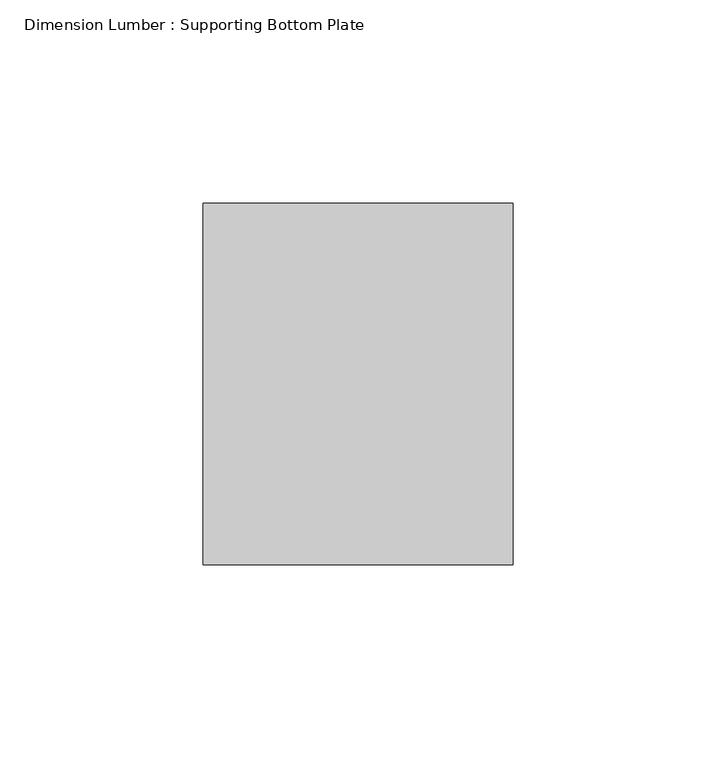
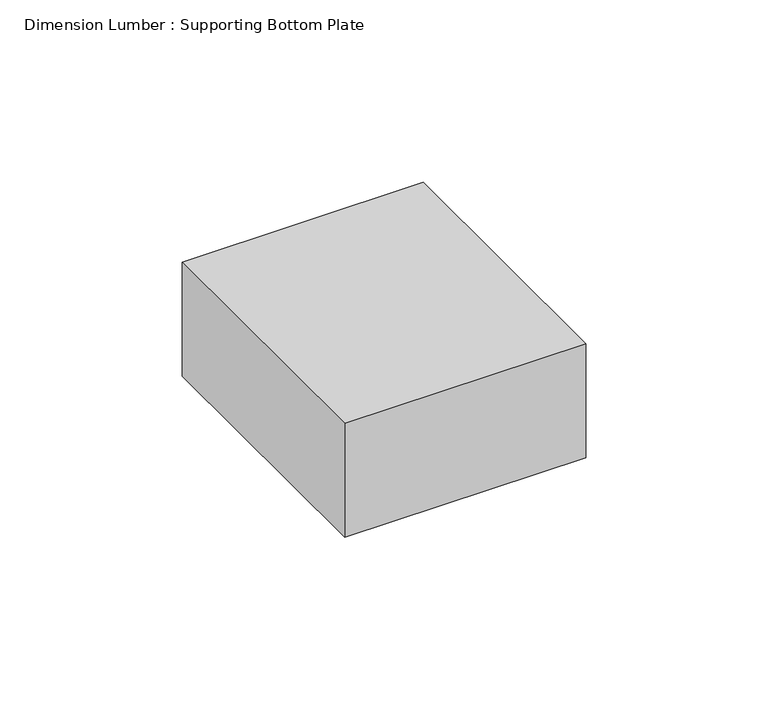
"""IFC4 building model written with IfcOpenShell, lengths in millimetres: beam geometry, Dimension Lumber : Supporting Bottom Plate."""

import ifcopenshell
import ifcopenshell.guid

model = None  # the IFC model being written
_history = None  # IfcOwnerHistory: only IFC2X3 demands one
_inside = {}  # id of a spatial element -> (the spatial element, [elements in it])
_under = {}  # id of a project, library or spatial element -> (it, [spatial elements below it])
_declared = {}  # id of a project -> (the project, [libraries it declares])
_typed = {}  # id of a type object -> (the type object, [elements of that type])
_made_of = {}  # id of a material, layer set ... -> (it, [elements and type objects made of it])


def new_model(schema):
    """Start an empty IFC model of exactly this schema.

    Asked for "IFC4X3", IfcOpenShell would pick the latest addendum, in which some entities
    have other attributes; the version numbers below select the first issue.
    IFC2X3 requires an IfcOwnerHistory on every rooted entity: one is made here for all.
    """
    global model, _history
    if schema == "IFC4X3":
        model = ifcopenshell.file(schema_version=(4, 3, 0, 0))
    else:
        model = ifcopenshell.file(schema=schema)
    _inside.clear()
    _under.clear()
    _declared.clear()
    _typed.clear()
    _made_of.clear()
    _history = None
    if model.schema == "IFC2X3":
        org = make("IfcOrganization", Name="unknown")
        user = make(
            "IfcPersonAndOrganization",
            ThePerson=make("IfcPerson", FamilyName="unknown"),
            TheOrganization=org,
        )
        app = make(
            "IfcApplication",
            ApplicationDeveloper=org,
            Version="unknown",
            ApplicationFullName="unknown",
            ApplicationIdentifier="unknown",
        )
        _history = make(
            "IfcOwnerHistory",
            OwningUser=user,
            OwningApplication=app,
            ChangeAction="ADDED",
            CreationDate=0,
        )
    return model


def make(cls, **values):
    """One entity of the class cls with the attributes given. An attribute that is None is left unset."""
    return model.create_entity(
        cls, **{name: value for name, value in values.items() if value is not None}
    )


def rooted(cls, **values):
    """An entity with a GlobalId (a new one), such as an element, a storey or a relation."""
    return make(cls, GlobalId=ifcopenshell.guid.new(), OwnerHistory=_history, **values)


def si_unit(unit_type, name, prefix=None):
    """IfcSIUnit, for example si_unit("LENGTHUNIT", "METRE", prefix="MILLI")."""
    return make("IfcSIUnit", UnitType=unit_type, Prefix=prefix, Name=name)


def assignment(units):
    """IfcUnitAssignment: the units of a project."""
    return None if units is None else make("IfcUnitAssignment", Units=units)


def point(xyz):
    """IfcCartesianPoint."""
    return None if xyz is None else make("IfcCartesianPoint", Coordinates=xyz)


def direction(xyz):
    """IfcDirection."""
    return None if xyz is None else make("IfcDirection", DirectionRatios=xyz)


def frame(location, z_axis=None, x_axis=None):
    """IfcAxis2Placement3D, a coordinate frame: its origin and axes. An axis left out is left unset."""
    return make(
        "IfcAxis2Placement3D",
        Location=point(location),
        Axis=direction(z_axis),
        RefDirection=direction(x_axis),
    )


def origin():
    """The frame at (0, 0, 0) with its axes left unset."""
    return frame((0.0, 0.0, 0.0))


def place(relative_to, where):
    """IfcLocalPlacement: puts the frame where relative to a parent placement (None: the world)."""
    return make(
        "IfcLocalPlacement", PlacementRelTo=relative_to, RelativePlacement=where
    )


def context(
    kind, dimensions, precision=None, world=None, true_north=None, identifier=None
):
    """IfcGeometricRepresentationContext, for example the 3D "Model" context."""
    return make(
        "IfcGeometricRepresentationContext",
        ContextIdentifier=identifier,
        ContextType=kind,
        CoordinateSpaceDimension=dimensions,
        Precision=precision,
        WorldCoordinateSystem=world,
        TrueNorth=true_north,
    )


def project(units=None, contexts=None):
    """IfcProject with its units and contexts."""
    return rooted(
        "IfcProject",
        Name="project",
        RepresentationContexts=contexts,
        UnitsInContext=assignment(units),
    )


def spatial(cls, under=None, at=None, **own):
    """A site, building, storey or space (cls), placed at a placement, below another one or the project."""
    s = rooted(cls, ObjectPlacement=at, **own)
    if under is not None:
        _under.setdefault(under.id(), (under, []))[1].append(s)
    return s


def polyline(points):
    """IfcPolyline through the points."""
    return make("IfcPolyline", Points=[point(p) for p in points])


def outline(outer, holes=None, kind="AREA"):
    """IfcArbitraryClosedProfileDef: a profile drawn as a closed curve; with holes, ...WithVoids."""
    if holes is None:
        return make("IfcArbitraryClosedProfileDef", ProfileType=kind, OuterCurve=outer)
    return make(
        "IfcArbitraryProfileDefWithVoids",
        ProfileType=kind,
        OuterCurve=outer,
        InnerCurves=holes,
    )


def extrude(swept, where, along, depth):
    """IfcExtrudedAreaSolid: the profile swept, set in the frame where, extruded along a direction by depth."""
    return make(
        "IfcExtrudedAreaSolid",
        SweptArea=swept,
        Position=where,
        ExtrudedDirection=direction(along),
        Depth=depth,
    )


def shape(context_of_items, identifier, shape_type, items):
    """IfcShapeRepresentation: the items that make up one representation, for example the "Body"."""
    return make(
        "IfcShapeRepresentation",
        ContextOfItems=context_of_items,
        RepresentationIdentifier=identifier,
        RepresentationType=shape_type,
        Items=items,
    )


def source(mapping_origin, context_of_items, identifier, shape_type, items):
    """IfcRepresentationMap: a shape defined once, which mapped items show again and again."""
    return make(
        "IfcRepresentationMap",
        MappingOrigin=mapping_origin,
        MappedRepresentation=shape(context_of_items, identifier, shape_type, items),
    )


def transform(
    local_origin,
    x_axis=None,
    y_axis=None,
    z_axis=None,
    scale=None,
    scale2=None,
    scale3=None,
    uniform=True,
):
    """IfcCartesianTransformationOperator3D, or its non-uniform kind. x_axis, y_axis, z_axis: its Axis1, 2, 3."""
    if uniform:
        return make(
            "IfcCartesianTransformationOperator3D",
            Axis1=direction(x_axis),
            Axis2=direction(y_axis),
            LocalOrigin=point(local_origin),
            Scale=scale,
            Axis3=direction(z_axis),
        )
    return make(
        "IfcCartesianTransformationOperator3DnonUniform",
        Axis1=direction(x_axis),
        Axis2=direction(y_axis),
        LocalOrigin=point(local_origin),
        Scale=scale,
        Axis3=direction(z_axis),
        Scale2=scale2,
        Scale3=scale3,
    )


def mapped(mapping_source, mapping_target):
    """IfcMappedItem: shows the shape of a source again, moved by a transform."""
    return make(
        "IfcMappedItem", MappingSource=mapping_source, MappingTarget=mapping_target
    )


def made_of(thing, what):
    """Note that an element or type object is made of a material, layer set ...; save() writes the relation."""
    if what is not None:
        _made_of.setdefault(what.id(), (what, []))[1].append(thing)
    return thing


def element(
    cls,
    number,
    at=None,
    inside=None,
    cuts=None,
    type_object=None,
    material=None,
    context=None,
    identifier="Body",
    shape_type=None,
    held_by="IfcProductDefinitionShape",
    body=None,
    shapes=None,
    **own,
):
    """One element of the class cls, such as IfcWall. Its Tag is "e" and its number.

    at: its placement. inside: the storey or other place that contains it. cuts: it is an
    opening in that element (IfcRelVoidsElement). A single representation is given by context,
    identifier, shape_type and body (its items); several are given by shapes. held_by: the class
    of the entity that holds the representations. save() writes the other relations.
    """
    e = rooted(cls, Tag="e%d" % number, ObjectPlacement=at, **own)
    if body is not None:
        shapes = [shape(context, identifier, shape_type, body)]
    if shapes is not None:
        e.Representation = make(held_by, Representations=shapes)
    if inside is not None:
        _inside.setdefault(inside.id(), (inside, []))[1].append(e)
    if cuts is not None:
        rooted(
            "IfcRelVoidsElement", RelatingBuildingElement=cuts, RelatedOpeningElement=e
        )
    if type_object is not None:
        _typed.setdefault(type_object.id(), (type_object, []))[1].append(e)
    return made_of(e, material)


def aggregate(whole, parts):
    """IfcRelAggregates: a whole, such as a stair, and the parts it consists of."""
    return rooted("IfcRelAggregates", RelatingObject=whole, RelatedObjects=parts)


def save(model, path):
    """Write the relations noted so far, then the file.

    IfcRelAggregates (storeys below a building ...), IfcRelContainedInSpatialStructure (elements
    in a storey), IfcRelDefinesByType, IfcRelAssociatesMaterial and IfcRelDeclares: one each for
    every whole, place, type object, material and project.
    """
    for whole, parts in _under.values():
        aggregate(whole, parts)
    for where, things in _inside.values():
        rooted(
            "IfcRelContainedInSpatialStructure",
            RelatedElements=things,
            RelatingStructure=where,
        )
    for kind, things in _typed.values():
        rooted("IfcRelDefinesByType", RelatedObjects=things, RelatingType=kind)
    for what, things in _made_of.values():
        rooted("IfcRelAssociatesMaterial", RelatedObjects=things, RelatingMaterial=what)
    for by, libraries in _declared.values():
        rooted("IfcRelDeclares", RelatingContext=by, RelatedDefinitions=libraries)
    model.write(path)


def dimension_lumber_supporting_bottom_plate_625eb92f(model_context):
    return source(origin(), model_context, "Body", "SweptSolid", [
        extrude(outline(polyline([(152.7017019, -44.45), (76.5017019, -44.45), (76.5017019, 44.45), (152.7017019, 44.45), (152.7017019, -44.45)])), frame((0.0, 0.0, -19.05), z_axis=(0.0, 0.0, 1.0), x_axis=(1.0, 0.0, 0.0)), (0.0, 0.0, 1.0), 38.1),
    ])


if __name__ == "__main__":
    model = new_model("IFC4")
    model_context = context("Model", 3, world=origin())
    ifc_project = project(units=[si_unit("LENGTHUNIT", "METRE", prefix="MILLI")], contexts=[model_context])
    site = spatial("IfcSite", under=ifc_project)
    building = spatial("IfcBuilding", under=site)
    placement = place(None, origin())
    dimension_lumber_supporting_bottom_plate_shape = dimension_lumber_supporting_bottom_plate_625eb92f(model_context)
    element("IfcBeam", 1, ObjectType="Dimension Lumber : Supporting Bottom Plate", at=placement, inside=building, context=model_context, shape_type="MappedRepresentation", body=[
        mapped(dimension_lumber_supporting_bottom_plate_shape, transform((0.0, 0.0, 0.0), x_axis=(1.0, 0.0, 0.0), y_axis=(0.0, 1.0, 0.0), z_axis=(0.0, 0.0, 1.0))),
    ])
    save(model, "model.ifc")

# Revit data of these elements
# Type "Dimension Lumber : Supporting Bottom Plate"
#   Assembly Code = "B10"
#   A = 0.0364583 SF
#   Length [instance default] = 5' - 0"
#   b = 0' - 3 1/2"
#   d = 0' - 1 1/2"
#   Structural Material [instance default] = Softwood, Lumber
# Element 1 (IfcBeam, "Dimension Lumber : Supporting Bottom Plate")
#   Structural Material = Douglas Fir #2
#   Materials on its faces: "Douglas Fir #2"
# Materials
#   "Softwood, Lumber": class "Wood", colour RGB 223 192 134, transparency 0, Description = "Pinus Echinata", Cost = 0
#   "Douglas Fir #2": class "Wood", colour RGB 223 192 134, transparency 0, Description = "Pinus Echinata", Cost = 0
